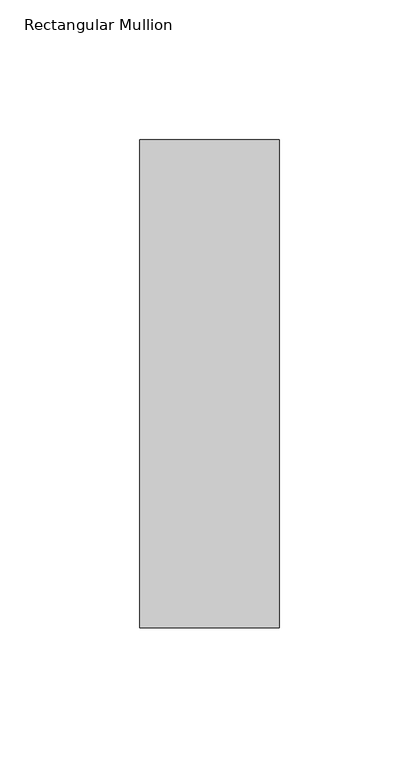
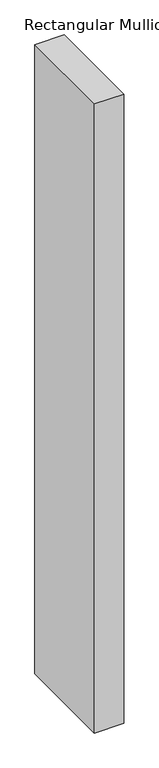
"""IFC4 building model written with IfcOpenShell, lengths in millimetres: member geometry, Rectangular Mullion : WWm-50x175-50mmOffset."""

import ifcopenshell
import ifcopenshell.guid

model = None  # the IFC model being written
_history = None  # IfcOwnerHistory: only IFC2X3 demands one
_inside = {}  # id of a spatial element -> (the spatial element, [elements in it])
_under = {}  # id of a project, library or spatial element -> (it, [spatial elements below it])
_declared = {}  # id of a project -> (the project, [libraries it declares])
_typed = {}  # id of a type object -> (the type object, [elements of that type])
_made_of = {}  # id of a material, layer set ... -> (it, [elements and type objects made of it])


def new_model(schema):
    """Start an empty IFC model of exactly this schema.

    Asked for "IFC4X3", IfcOpenShell would pick the latest addendum, in which some entities
    have other attributes; the version numbers below select the first issue.
    IFC2X3 requires an IfcOwnerHistory on every rooted entity: one is made here for all.
    """
    global model, _history
    if schema == "IFC4X3":
        model = ifcopenshell.file(schema_version=(4, 3, 0, 0))
    else:
        model = ifcopenshell.file(schema=schema)
    _inside.clear()
    _under.clear()
    _declared.clear()
    _typed.clear()
    _made_of.clear()
    _history = None
    if model.schema == "IFC2X3":
        org = make("IfcOrganization", Name="unknown")
        user = make(
            "IfcPersonAndOrganization",
            ThePerson=make("IfcPerson", FamilyName="unknown"),
            TheOrganization=org,
        )
        app = make(
            "IfcApplication",
            ApplicationDeveloper=org,
            Version="unknown",
            ApplicationFullName="unknown",
            ApplicationIdentifier="unknown",
        )
        _history = make(
            "IfcOwnerHistory",
            OwningUser=user,
            OwningApplication=app,
            ChangeAction="ADDED",
            CreationDate=0,
        )
    return model


def make(cls, **values):
    """One entity of the class cls with the attributes given. An attribute that is None is left unset."""
    return model.create_entity(
        cls, **{name: value for name, value in values.items() if value is not None}
    )


def rooted(cls, **values):
    """An entity with a GlobalId (a new one), such as an element, a storey or a relation."""
    return make(cls, GlobalId=ifcopenshell.guid.new(), OwnerHistory=_history, **values)


def si_unit(unit_type, name, prefix=None):
    """IfcSIUnit, for example si_unit("LENGTHUNIT", "METRE", prefix="MILLI")."""
    return make("IfcSIUnit", UnitType=unit_type, Prefix=prefix, Name=name)


def assignment(units):
    """IfcUnitAssignment: the units of a project."""
    return None if units is None else make("IfcUnitAssignment", Units=units)


def point(xyz):
    """IfcCartesianPoint."""
    return None if xyz is None else make("IfcCartesianPoint", Coordinates=xyz)


def direction(xyz):
    """IfcDirection."""
    return None if xyz is None else make("IfcDirection", DirectionRatios=xyz)


def frame(location, z_axis=None, x_axis=None):
    """IfcAxis2Placement3D, a coordinate frame: its origin and axes. An axis left out is left unset."""
    return make(
        "IfcAxis2Placement3D",
        Location=point(location),
        Axis=direction(z_axis),
        RefDirection=direction(x_axis),
    )


def origin():
    """The frame at (0, 0, 0) with its axes left unset."""
    return frame((0.0, 0.0, 0.0))


def place(relative_to, where):
    """IfcLocalPlacement: puts the frame where relative to a parent placement (None: the world)."""
    return make(
        "IfcLocalPlacement", PlacementRelTo=relative_to, RelativePlacement=where
    )


def context(
    kind, dimensions, precision=None, world=None, true_north=None, identifier=None
):
    """IfcGeometricRepresentationContext, for example the 3D "Model" context."""
    return make(
        "IfcGeometricRepresentationContext",
        ContextIdentifier=identifier,
        ContextType=kind,
        CoordinateSpaceDimension=dimensions,
        Precision=precision,
        WorldCoordinateSystem=world,
        TrueNorth=true_north,
    )


def project(units=None, contexts=None):
    """IfcProject with its units and contexts."""
    return rooted(
        "IfcProject",
        Name="project",
        RepresentationContexts=contexts,
        UnitsInContext=assignment(units),
    )


def spatial(cls, under=None, at=None, **own):
    """A site, building, storey or space (cls), placed at a placement, below another one or the project."""
    s = rooted(cls, ObjectPlacement=at, **own)
    if under is not None:
        _under.setdefault(under.id(), (under, []))[1].append(s)
    return s


def polyline(points):
    """IfcPolyline through the points."""
    return make("IfcPolyline", Points=[point(p) for p in points])


def outline(outer, holes=None, kind="AREA"):
    """IfcArbitraryClosedProfileDef: a profile drawn as a closed curve; with holes, ...WithVoids."""
    if holes is None:
        return make("IfcArbitraryClosedProfileDef", ProfileType=kind, OuterCurve=outer)
    return make(
        "IfcArbitraryProfileDefWithVoids",
        ProfileType=kind,
        OuterCurve=outer,
        InnerCurves=holes,
    )


def extrude(swept, where, along, depth):
    """IfcExtrudedAreaSolid: the profile swept, set in the frame where, extruded along a direction by depth."""
    return make(
        "IfcExtrudedAreaSolid",
        SweptArea=swept,
        Position=where,
        ExtrudedDirection=direction(along),
        Depth=depth,
    )


def shape(context_of_items, identifier, shape_type, items):
    """IfcShapeRepresentation: the items that make up one representation, for example the "Body"."""
    return make(
        "IfcShapeRepresentation",
        ContextOfItems=context_of_items,
        RepresentationIdentifier=identifier,
        RepresentationType=shape_type,
        Items=items,
    )


def source(mapping_origin, context_of_items, identifier, shape_type, items):
    """IfcRepresentationMap: a shape defined once, which mapped items show again and again."""
    return make(
        "IfcRepresentationMap",
        MappingOrigin=mapping_origin,
        MappedRepresentation=shape(context_of_items, identifier, shape_type, items),
    )


def transform(
    local_origin,
    x_axis=None,
    y_axis=None,
    z_axis=None,
    scale=None,
    scale2=None,
    scale3=None,
    uniform=True,
):
    """IfcCartesianTransformationOperator3D, or its non-uniform kind. x_axis, y_axis, z_axis: its Axis1, 2, 3."""
    if uniform:
        return make(
            "IfcCartesianTransformationOperator3D",
            Axis1=direction(x_axis),
            Axis2=direction(y_axis),
            LocalOrigin=point(local_origin),
            Scale=scale,
            Axis3=direction(z_axis),
        )
    return make(
        "IfcCartesianTransformationOperator3DnonUniform",
        Axis1=direction(x_axis),
        Axis2=direction(y_axis),
        LocalOrigin=point(local_origin),
        Scale=scale,
        Axis3=direction(z_axis),
        Scale2=scale2,
        Scale3=scale3,
    )


def mapped(mapping_source, mapping_target):
    """IfcMappedItem: shows the shape of a source again, moved by a transform."""
    return make(
        "IfcMappedItem", MappingSource=mapping_source, MappingTarget=mapping_target
    )


def made_of(thing, what):
    """Note that an element or type object is made of a material, layer set ...; save() writes the relation."""
    if what is not None:
        _made_of.setdefault(what.id(), (what, []))[1].append(thing)
    return thing


def element(
    cls,
    number,
    at=None,
    inside=None,
    cuts=None,
    type_object=None,
    material=None,
    context=None,
    identifier="Body",
    shape_type=None,
    held_by="IfcProductDefinitionShape",
    body=None,
    shapes=None,
    **own,
):
    """One element of the class cls, such as IfcWall. Its Tag is "e" and its number.

    at: its placement. inside: the storey or other place that contains it. cuts: it is an
    opening in that element (IfcRelVoidsElement). A single representation is given by context,
    identifier, shape_type and body (its items); several are given by shapes. held_by: the class
    of the entity that holds the representations. save() writes the other relations.
    """
    e = rooted(cls, Tag="e%d" % number, ObjectPlacement=at, **own)
    if body is not None:
        shapes = [shape(context, identifier, shape_type, body)]
    if shapes is not None:
        e.Representation = make(held_by, Representations=shapes)
    if inside is not None:
        _inside.setdefault(inside.id(), (inside, []))[1].append(e)
    if cuts is not None:
        rooted(
            "IfcRelVoidsElement", RelatingBuildingElement=cuts, RelatedOpeningElement=e
        )
    if type_object is not None:
        _typed.setdefault(type_object.id(), (type_object, []))[1].append(e)
    return made_of(e, material)


def aggregate(whole, parts):
    """IfcRelAggregates: a whole, such as a stair, and the parts it consists of."""
    return rooted("IfcRelAggregates", RelatingObject=whole, RelatedObjects=parts)


def save(model, path):
    """Write the relations noted so far, then the file.

    IfcRelAggregates (storeys below a building ...), IfcRelContainedInSpatialStructure (elements
    in a storey), IfcRelDefinesByType, IfcRelAssociatesMaterial and IfcRelDeclares: one each for
    every whole, place, type object, material and project.
    """
    for whole, parts in _under.values():
        aggregate(whole, parts)
    for where, things in _inside.values():
        rooted(
            "IfcRelContainedInSpatialStructure",
            RelatedElements=things,
            RelatingStructure=where,
        )
    for kind, things in _typed.values():
        rooted("IfcRelDefinesByType", RelatedObjects=things, RelatingType=kind)
    for what, things in _made_of.values():
        rooted("IfcRelAssociatesMaterial", RelatedObjects=things, RelatingMaterial=what)
    for by, libraries in _declared.values():
        rooted("IfcRelDeclares", RelatingContext=by, RelatedDefinitions=libraries)
    model.write(path)


def rectangular_mullion_6e49eaec(model_context):
    return source(origin(), model_context, "Body", "SweptSolid", [
        extrude(outline(polyline([(0.0, 87.5), (0.0, -87.5), (-50.0, -87.5), (-50.0, 87.5), (0.0, 87.5)])), frame((0.0, 0.0, -1130.0), z_axis=(0.0, 0.0, 1.0), x_axis=(1.0, 0.0, 0.0)), (0.0, 0.0, 1.0), 1130.0),
    ])


if __name__ == "__main__":
    model = new_model("IFC4")
    model_context = context("Model", 3, world=origin())
    ifc_project = project(units=[si_unit("LENGTHUNIT", "METRE", prefix="MILLI")], contexts=[model_context])
    site = spatial("IfcSite", under=ifc_project)
    building = spatial("IfcBuilding", under=site)
    placement = place(None, origin())
    rectangular_mullion_shape = rectangular_mullion_6e49eaec(model_context)
    element("IfcMember", 1, ObjectType="Rectangular Mullion : WWm-50x175-50mmOffset", at=placement, inside=building, context=model_context, shape_type="MappedRepresentation", body=[
        mapped(rectangular_mullion_shape, transform((0.0, 0.0, 0.0), x_axis=(1.0, 0.0, 0.0), y_axis=(0.0, 1.0, 0.0), z_axis=(0.0, 0.0, 1.0))),
    ])
    save(model, "model.ifc")

# Revit data of these elements
# Type "Rectangular Mullion : WWm-50x175-50mmOffset"
#   built-in parameter 1007304 = 0.574147 (stored number, unit not read)
#   built-in parameter 1007301 = 0.082021 (stored number, unit not read)
#   built-in parameter 1007300 = 0.082021 (stored number, unit not read)
# Element 1 (IfcMember, "Rectangular Mullion : WWm-50x175-50mmOffset")
#   Materials on its faces: "WW-EC-RGB-Mullion"
# Materials
#   "WW-EC-RGB-Mullion": class "Generic", colour RGB 255 255 255, transparency 0, Comments = "If region requests black mullions, switch asset color to RGB 25-25-25", Description = "Generic Color", Cost = 0
